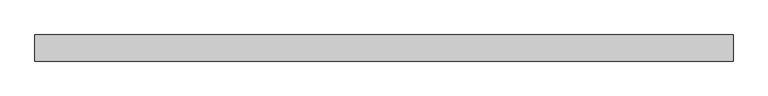
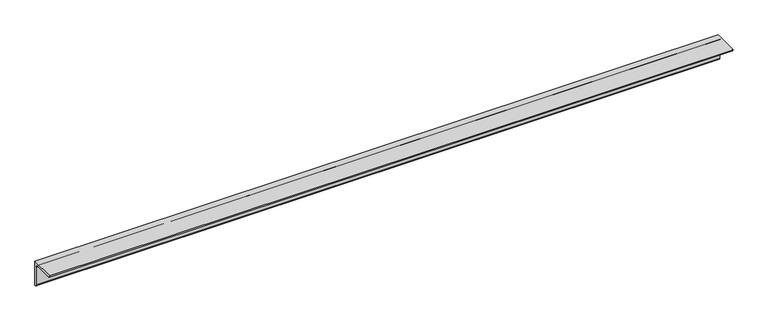
"""IFC4 building model written with IfcOpenShell, lengths in millimetres: member geometry, 0912_Steel Framing_L-KSD3502 : H_SB_AR_S03_L-130x130x12_HBR3."""

import ifcopenshell
import ifcopenshell.guid

model = None  # the IFC model being written
_history = None  # IfcOwnerHistory: only IFC2X3 demands one
_inside = {}  # id of a spatial element -> (the spatial element, [elements in it])
_under = {}  # id of a project, library or spatial element -> (it, [spatial elements below it])
_declared = {}  # id of a project -> (the project, [libraries it declares])
_typed = {}  # id of a type object -> (the type object, [elements of that type])
_made_of = {}  # id of a material, layer set ... -> (it, [elements and type objects made of it])


def new_model(schema):
    """Start an empty IFC model of exactly this schema.

    Asked for "IFC4X3", IfcOpenShell would pick the latest addendum, in which some entities
    have other attributes; the version numbers below select the first issue.
    IFC2X3 requires an IfcOwnerHistory on every rooted entity: one is made here for all.
    """
    global model, _history
    if schema == "IFC4X3":
        model = ifcopenshell.file(schema_version=(4, 3, 0, 0))
    else:
        model = ifcopenshell.file(schema=schema)
    _inside.clear()
    _under.clear()
    _declared.clear()
    _typed.clear()
    _made_of.clear()
    _history = None
    if model.schema == "IFC2X3":
        org = make("IfcOrganization", Name="unknown")
        user = make(
            "IfcPersonAndOrganization",
            ThePerson=make("IfcPerson", FamilyName="unknown"),
            TheOrganization=org,
        )
        app = make(
            "IfcApplication",
            ApplicationDeveloper=org,
            Version="unknown",
            ApplicationFullName="unknown",
            ApplicationIdentifier="unknown",
        )
        _history = make(
            "IfcOwnerHistory",
            OwningUser=user,
            OwningApplication=app,
            ChangeAction="ADDED",
            CreationDate=0,
        )
    return model


def make(cls, **values):
    """One entity of the class cls with the attributes given. An attribute that is None is left unset."""
    return model.create_entity(
        cls, **{name: value for name, value in values.items() if value is not None}
    )


def rooted(cls, **values):
    """An entity with a GlobalId (a new one), such as an element, a storey or a relation."""
    return make(cls, GlobalId=ifcopenshell.guid.new(), OwnerHistory=_history, **values)


def si_unit(unit_type, name, prefix=None):
    """IfcSIUnit, for example si_unit("LENGTHUNIT", "METRE", prefix="MILLI")."""
    return make("IfcSIUnit", UnitType=unit_type, Prefix=prefix, Name=name)


def assignment(units):
    """IfcUnitAssignment: the units of a project."""
    return None if units is None else make("IfcUnitAssignment", Units=units)


def point(xyz):
    """IfcCartesianPoint."""
    return None if xyz is None else make("IfcCartesianPoint", Coordinates=xyz)


def direction(xyz):
    """IfcDirection."""
    return None if xyz is None else make("IfcDirection", DirectionRatios=xyz)


def frame(location, z_axis=None, x_axis=None):
    """IfcAxis2Placement3D, a coordinate frame: its origin and axes. An axis left out is left unset."""
    return make(
        "IfcAxis2Placement3D",
        Location=point(location),
        Axis=direction(z_axis),
        RefDirection=direction(x_axis),
    )


def frame_2d(location, x_axis=None):
    """IfcAxis2Placement2D, a coordinate frame in the plane: its origin and x axis."""
    return make(
        "IfcAxis2Placement2D", Location=point(location), RefDirection=direction(x_axis)
    )


def origin():
    """The frame at (0, 0, 0) with its axes left unset."""
    return frame((0.0, 0.0, 0.0))


def place(relative_to, where):
    """IfcLocalPlacement: puts the frame where relative to a parent placement (None: the world)."""
    return make(
        "IfcLocalPlacement", PlacementRelTo=relative_to, RelativePlacement=where
    )


def context(
    kind, dimensions, precision=None, world=None, true_north=None, identifier=None
):
    """IfcGeometricRepresentationContext, for example the 3D "Model" context."""
    return make(
        "IfcGeometricRepresentationContext",
        ContextIdentifier=identifier,
        ContextType=kind,
        CoordinateSpaceDimension=dimensions,
        Precision=precision,
        WorldCoordinateSystem=world,
        TrueNorth=true_north,
    )


def project(units=None, contexts=None):
    """IfcProject with its units and contexts."""
    return rooted(
        "IfcProject",
        Name="project",
        RepresentationContexts=contexts,
        UnitsInContext=assignment(units),
    )


def spatial(cls, under=None, at=None, **own):
    """A site, building, storey or space (cls), placed at a placement, below another one or the project."""
    s = rooted(cls, ObjectPlacement=at, **own)
    if under is not None:
        _under.setdefault(under.id(), (under, []))[1].append(s)
    return s


def polyline(points):
    """IfcPolyline through the points."""
    return make("IfcPolyline", Points=[point(p) for p in points])


def circle_curve(where, radius):
    """IfcCircle in the frame where."""
    return make("IfcCircle", Position=where, Radius=radius)


def trimmed(basis, trim1, trim2, sense, master):
    """IfcTrimmedCurve: the piece of a basis curve between two trims."""
    return make(
        "IfcTrimmedCurve",
        BasisCurve=basis,
        Trim1=trim1,
        Trim2=trim2,
        SenseAgreement=sense,
        MasterRepresentation=master,
    )


def segment(curve, same_sense, transition):
    """IfcCompositeCurveSegment."""
    return make(
        "IfcCompositeCurveSegment",
        Transition=transition,
        SameSense=same_sense,
        ParentCurve=curve,
    )


def composite_curve(segments, self_intersect=None):
    """IfcCompositeCurve: segments joined end to end."""
    return make("IfcCompositeCurve", Segments=segments, SelfIntersect=self_intersect)


def outline(outer, holes=None, kind="AREA"):
    """IfcArbitraryClosedProfileDef: a profile drawn as a closed curve; with holes, ...WithVoids."""
    if holes is None:
        return make("IfcArbitraryClosedProfileDef", ProfileType=kind, OuterCurve=outer)
    return make(
        "IfcArbitraryProfileDefWithVoids",
        ProfileType=kind,
        OuterCurve=outer,
        InnerCurves=holes,
    )


def extrude(swept, where, along, depth):
    """IfcExtrudedAreaSolid: the profile swept, set in the frame where, extruded along a direction by depth."""
    return make(
        "IfcExtrudedAreaSolid",
        SweptArea=swept,
        Position=where,
        ExtrudedDirection=direction(along),
        Depth=depth,
    )


def shape(context_of_items, identifier, shape_type, items):
    """IfcShapeRepresentation: the items that make up one representation, for example the "Body"."""
    return make(
        "IfcShapeRepresentation",
        ContextOfItems=context_of_items,
        RepresentationIdentifier=identifier,
        RepresentationType=shape_type,
        Items=items,
    )


def source(mapping_origin, context_of_items, identifier, shape_type, items):
    """IfcRepresentationMap: a shape defined once, which mapped items show again and again."""
    return make(
        "IfcRepresentationMap",
        MappingOrigin=mapping_origin,
        MappedRepresentation=shape(context_of_items, identifier, shape_type, items),
    )


def transform(
    local_origin,
    x_axis=None,
    y_axis=None,
    z_axis=None,
    scale=None,
    scale2=None,
    scale3=None,
    uniform=True,
):
    """IfcCartesianTransformationOperator3D, or its non-uniform kind. x_axis, y_axis, z_axis: its Axis1, 2, 3."""
    if uniform:
        return make(
            "IfcCartesianTransformationOperator3D",
            Axis1=direction(x_axis),
            Axis2=direction(y_axis),
            LocalOrigin=point(local_origin),
            Scale=scale,
            Axis3=direction(z_axis),
        )
    return make(
        "IfcCartesianTransformationOperator3DnonUniform",
        Axis1=direction(x_axis),
        Axis2=direction(y_axis),
        LocalOrigin=point(local_origin),
        Scale=scale,
        Axis3=direction(z_axis),
        Scale2=scale2,
        Scale3=scale3,
    )


def mapped(mapping_source, mapping_target):
    """IfcMappedItem: shows the shape of a source again, moved by a transform."""
    return make(
        "IfcMappedItem", MappingSource=mapping_source, MappingTarget=mapping_target
    )


def made_of(thing, what):
    """Note that an element or type object is made of a material, layer set ...; save() writes the relation."""
    if what is not None:
        _made_of.setdefault(what.id(), (what, []))[1].append(thing)
    return thing


def element(
    cls,
    number,
    at=None,
    inside=None,
    cuts=None,
    type_object=None,
    material=None,
    context=None,
    identifier="Body",
    shape_type=None,
    held_by="IfcProductDefinitionShape",
    body=None,
    shapes=None,
    **own,
):
    """One element of the class cls, such as IfcWall. Its Tag is "e" and its number.

    at: its placement. inside: the storey or other place that contains it. cuts: it is an
    opening in that element (IfcRelVoidsElement). A single representation is given by context,
    identifier, shape_type and body (its items); several are given by shapes. held_by: the class
    of the entity that holds the representations. save() writes the other relations.
    """
    e = rooted(cls, Tag="e%d" % number, ObjectPlacement=at, **own)
    if body is not None:
        shapes = [shape(context, identifier, shape_type, body)]
    if shapes is not None:
        e.Representation = make(held_by, Representations=shapes)
    if inside is not None:
        _inside.setdefault(inside.id(), (inside, []))[1].append(e)
    if cuts is not None:
        rooted(
            "IfcRelVoidsElement", RelatingBuildingElement=cuts, RelatedOpeningElement=e
        )
    if type_object is not None:
        _typed.setdefault(type_object.id(), (type_object, []))[1].append(e)
    return made_of(e, material)


def aggregate(whole, parts):
    """IfcRelAggregates: a whole, such as a stair, and the parts it consists of."""
    return rooted("IfcRelAggregates", RelatingObject=whole, RelatedObjects=parts)


def save(model, path):
    """Write the relations noted so far, then the file.

    IfcRelAggregates (storeys below a building ...), IfcRelContainedInSpatialStructure (elements
    in a storey), IfcRelDefinesByType, IfcRelAssociatesMaterial and IfcRelDeclares: one each for
    every whole, place, type object, material and project.
    """
    for whole, parts in _under.values():
        aggregate(whole, parts)
    for where, things in _inside.values():
        rooted(
            "IfcRelContainedInSpatialStructure",
            RelatedElements=things,
            RelatingStructure=where,
        )
    for kind, things in _typed.values():
        rooted("IfcRelDefinesByType", RelatedObjects=things, RelatingType=kind)
    for what, things in _made_of.values():
        rooted("IfcRelAssociatesMaterial", RelatedObjects=things, RelatingMaterial=what)
    for by, libraries in _declared.values():
        rooted("IfcRelDeclares", RelatingContext=by, RelatedDefinitions=libraries)
    model.write(path)


def member_46ab37a3(model_context):
    return source(origin(), model_context, "Body", "SweptSolid", [
        extrude(outline(composite_curve([segment(polyline([(36.4, 36.4), (36.4, -93.6)]), True, "CONTINUOUS"), segment(trimmed(circle_curve(frame_2d((36.4, -81.6)), 12.0), [point((36.4, -93.6))], [point((24.4, -81.6))], False, "CARTESIAN"), True, "CONTINUOUS"), segment(polyline([(24.4, -81.6), (24.4, 12.4)]), True, "CONTINUOUS"), segment(trimmed(circle_curve(frame_2d((12.4, 12.4)), 12.0), [point((24.4, 12.4))], [point((12.4, 24.4))], True, "CARTESIAN"), True, "CONTINUOUS"), segment(polyline([(12.4, 24.4), (-81.6, 24.4)]), True, "CONTINUOUS"), segment(trimmed(circle_curve(frame_2d((-81.6, 36.4)), 12.0), [point((-81.6, 24.4))], [point((-93.6, 36.4))], False, "CARTESIAN"), True, "CONTINUOUS"), segment(polyline([(-93.6, 36.4), (36.4, 36.4)]), True, "CONTINUOUS")], self_intersect=False)), frame((-1750.5663611, 0.0, 0.0), z_axis=(1.0, 0.0, 0.0), x_axis=(0.0, 1.0, 0.0)), (0.0, 0.0, 1.0), 3476.5545794),
    ])


if __name__ == "__main__":
    model = new_model("IFC4")
    model_context = context("Model", 3, world=origin())
    ifc_project = project(units=[si_unit("LENGTHUNIT", "METRE", prefix="MILLI")], contexts=[model_context])
    site = spatial("IfcSite", under=ifc_project)
    building = spatial("IfcBuilding", under=site)
    placement = place(None, origin())
    member_shape = member_46ab37a3(model_context)
    element("IfcMember", 1, ObjectType="0912_Steel Framing_L-KSD3502 : H_SB_AR_S03_L-130x130x12_HBR3", at=placement, inside=building, context=model_context, shape_type="MappedRepresentation", body=[
        mapped(member_shape, transform((0.0, 0.0, 0.0), x_axis=(1.0, 0.0, 0.0), y_axis=(0.0, 1.0, 0.0), z_axis=(0.0, 0.0, 1.0))),
    ])
    save(model, "model.ifc")

# Revit data of these elements
# Type "0912_Steel Framing_L-KSD3502 : H_SB_AR_S03_L-130x130x12_HBR3"
#   k = 25 mm
#   Perimeter = 0.52 m²/m
#   Nominal Weight = 23.40 kgf/m
#   Length [instance default] = 1000 mm
#   b = 130 mm
#   d = 130 mm
#   t = 12 mm
#   x = 36.4 mm
#   y = 36.4 mm
#   A = 2976.00 m²
#   Structural Material [instance default] = Steel, 45-345
# Element 1 (IfcMember, "0912_Steel Framing_L-KSD3502 : H_SB_AR_S03_L-130x130x12_HBR3")
#   Structural Material = Steel ASTM A36
#   Materials on its faces: "Steel ASTM A36"
# Materials
#   "Steel, 45-345": class "Metal", colour RGB 189 187 185, transparency 0, Description = "Steel 345 MPa", Cost = 0
#   "Steel ASTM A36": class "Metal", colour RGB 199 199 199, transparency 0, Description = "Structural steel, ASTM A36 Grade B, mill finish", Cost = 0
